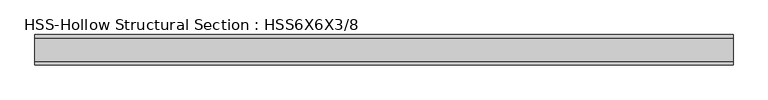
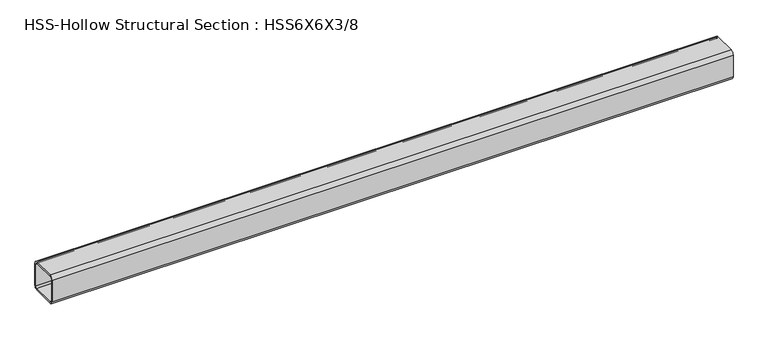
"""IFC4 building model written with IfcOpenShell, lengths in millimetres: beam geometry, HSS-Hollow Structural Section : HSS6X6X3/8."""

from ifc_helpers import new_model, si_unit, point, frame, frame_2d, origin, place, context, project, spatial, polyline, circle_curve, trimmed, segment, composite_curve, outline, extrude, source, transform, mapped, element, save


def hss_hollow_structural_section_hss6x6x3_8_4897b778(model_context):
    return source(origin(), model_context, "Body", "SweptSolid", [
        extrude(outline(composite_curve([segment(polyline([(76.2, 58.4708), (76.2, -58.4708)]), True, "CONTINUOUS"), segment(trimmed(circle_curve(frame_2d((58.4708, -58.4708)), 17.7292), [point((76.2, -58.4708))], [point((58.4708, -76.2))], False, "CARTESIAN"), True, "CONTINUOUS"), segment(polyline([(58.4708, -76.2), (-58.4708, -76.2)]), True, "CONTINUOUS"), segment(trimmed(circle_curve(frame_2d((-58.4708, -58.4708)), 17.7292), [point((-58.4708, -76.2))], [point((-76.2, -58.4708))], False, "CARTESIAN"), True, "CONTINUOUS"), segment(polyline([(-76.2, -58.4708), (-76.2, 58.4708)]), True, "CONTINUOUS"), segment(trimmed(circle_curve(frame_2d((-58.4708, 58.4708)), 17.7292), [point((-76.2, 58.4708))], [point((-58.4708, 76.2))], False, "CARTESIAN"), True, "CONTINUOUS"), segment(polyline([(-58.4708, 76.2), (58.4708, 76.2)]), True, "CONTINUOUS"), segment(trimmed(circle_curve(frame_2d((58.4708, 58.4708)), 17.7292), [point((58.4708, 76.2))], [point((76.2, 58.4708))], False, "CARTESIAN"), True, "CONTINUOUS")], self_intersect=False), holes=[composite_curve([segment(trimmed(circle_curve(frame_2d((-58.4708, 58.4708)), 8.8646), [point((-58.4708, 67.3354))], [point((-67.3354, 58.4708))], True, "CARTESIAN"), True, "CONTINUOUS"), segment(polyline([(-67.3354, 58.4708), (-67.3354, -58.4708)]), True, "CONTINUOUS"), segment(trimmed(circle_curve(frame_2d((-58.4708, -58.4708)), 8.8646), [point((-67.3354, -58.4708))], [point((-58.4708, -67.3354))], True, "CARTESIAN"), True, "CONTINUOUS"), segment(polyline([(-58.4708, -67.3354), (58.4708, -67.3354)]), True, "CONTINUOUS"), segment(trimmed(circle_curve(frame_2d((58.4708, -58.4708)), 8.8646), [point((58.4708, -67.3354))], [point((67.3354, -58.4708))], True, "CARTESIAN"), True, "CONTINUOUS"), segment(polyline([(67.3354, -58.4708), (67.3354, 58.4708)]), True, "CONTINUOUS"), segment(trimmed(circle_curve(frame_2d((58.4708, 58.4708)), 8.8646), [point((67.3354, 58.4708))], [point((58.4708, 67.3354))], True, "CARTESIAN"), True, "CONTINUOUS"), segment(polyline([(58.4708, 67.3354), (-58.4708, 67.3354)]), True, "CONTINUOUS")], self_intersect=False)]), frame((-1765.3, 0.0, 0.0), z_axis=(1.0, 0.0, 0.0), x_axis=(0.0, 1.0, 0.0)), (0.0, 0.0, 1.0), 3499.4799048),
    ])


if __name__ == "__main__":
    model = new_model("IFC4")
    model_context = context("Model", 3, world=origin())
    ifc_project = project(units=[si_unit("LENGTHUNIT", "METRE", prefix="MILLI")], contexts=[model_context])
    site = spatial("IfcSite", under=ifc_project)
    building = spatial("IfcBuilding", under=site)
    placement = place(None, origin())
    hss_hollow_structural_section_hss6x6x3_8_shape = hss_hollow_structural_section_hss6x6x3_8_4897b778(model_context)
    element("IfcBeam", 1, ObjectType="HSS-Hollow Structural Section : HSS6X6X3/8", at=placement, inside=building, context=model_context, shape_type="MappedRepresentation", body=[
        mapped(hss_hollow_structural_section_hss6x6x3_8_shape, transform((0.0, 0.0, 0.0), x_axis=(1.0, 0.0, 0.0), y_axis=(0.0, 1.0, 0.0), z_axis=(0.0, 0.0, 1.0))),
    ])
    save(model, "model.ifc")

# Revit data of these elements
# Type "HSS-Hollow Structural Section : HSS6X6X3/8"
#   Assembly Code = "B10"
#   Shape = "Square"
#   W = 27.4
#   Ht = 0' - 6"
#   Length [instance default] = 5' - 0"
#   b = 0' - 6"
#   kr = 0' - 0.698"
#   t = 0' - 0.349"
#   A = 0.0526389 SF
#   Structural Material [instance default] = Steel ASTM A500, Grade B, Rectangular and Square
# Element 1 (IfcBeam, "HSS-Hollow Structural Section : HSS6X6X3/8")
#   Materials on its faces: "Steel ASTM A500, Grade B, Rectangular and Square"
# Materials
#   "Steel ASTM A500, Grade B, Rectangular and Square": class "Metal", colour RGB 199 199 199, transparency 0, Description = "Carbon steel", Cost = 0
